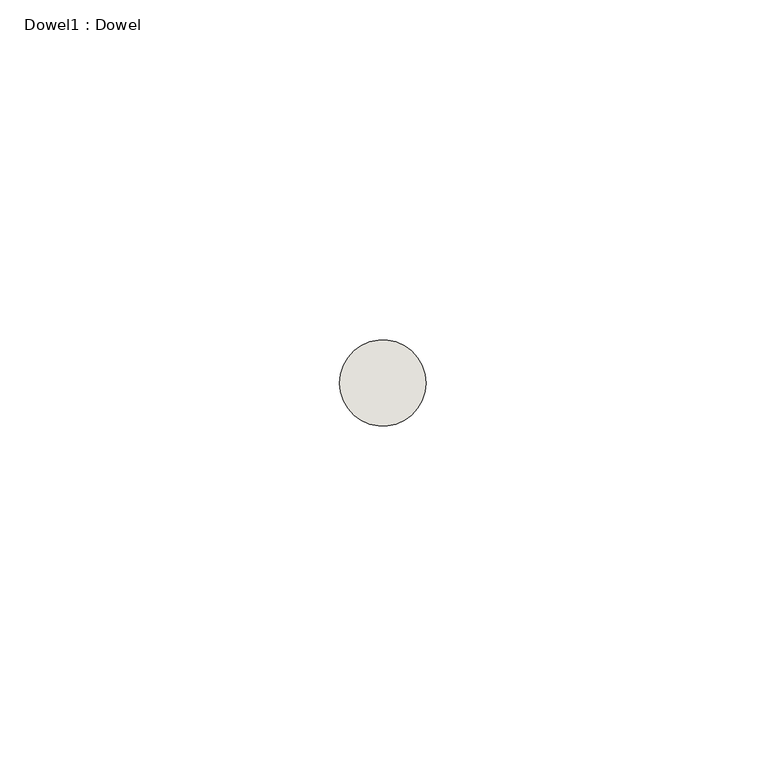
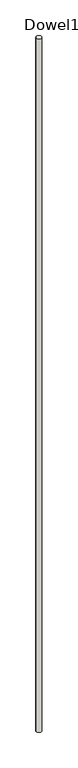
"""IFC4 building model written with IfcOpenShell, lengths in millimetres: wall geometry, Dowel1 : Dowel."""

from ifc_helpers import new_model, si_unit, point, frame, frame_2d, origin, place, context, project, spatial, circle_curve, trimmed, segment, composite_curve, outline, extrude, source, transform, mapped, element, save


def dowel1_dowel_b33121e9(model_context):
    return source(origin(), model_context, "Body", "SweptSolid", [
        extrude(outline(composite_curve([segment(trimmed(circle_curve(frame_2d((430101.375, 408.78125)), 6.35), [point((430095.025, 408.78125))], [point((430107.725, 408.78125))], False, "CARTESIAN"), True, "CONTINUOUS"), segment(trimmed(circle_curve(frame_2d((430101.375, 408.78125)), 6.35), [point((430107.725, 408.78125))], [point((430095.025, 408.78125))], False, "CARTESIAN"), True, "CONTINUOUS")], self_intersect=False)), frame((0.0, 0.0, 101.6), z_axis=(0.0, 0.0, 1.0), x_axis=(1.0, 0.0, 0.0)), (0.0, 0.0, 1.0), 1854.2),
    ])


if __name__ == "__main__":
    model = new_model("IFC4")
    model_context = context("Model", 3, world=origin())
    ifc_project = project(units=[si_unit("LENGTHUNIT", "METRE", prefix="MILLI")], contexts=[model_context])
    site = spatial("IfcSite", under=ifc_project)
    building = spatial("IfcBuilding", under=site)
    placement = place(None, origin())
    dowel1_dowel_shape = dowel1_dowel_b33121e9(model_context)
    element("IfcWall", 1, ObjectType="Dowel1 : Dowel", at=placement, inside=building, context=model_context, shape_type="MappedRepresentation", body=[
        mapped(dowel1_dowel_shape, transform((0.0, 0.0, 0.0), x_axis=(1.0, 0.0, 0.0), y_axis=(0.0, 1.0, 0.0), z_axis=(0.0, 0.0, 1.0))),
    ])
    save(model, "model.ifc")

# Revit data of these elements
# Element 1 (IfcWall, "Dowel1 : Dowel")
#   Materials on its faces: "6\" CMU WALL W/#4 VERT. BARS AT 32\" O.C. (TYP.)"
# Materials
#   "6\" CMU WALL W/#4 VERT. BARS AT 32\" O.C. (TYP.)": class "Generic", colour RGB 255 255 255, transparency 0, Cost = 0
